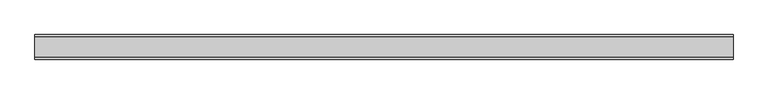
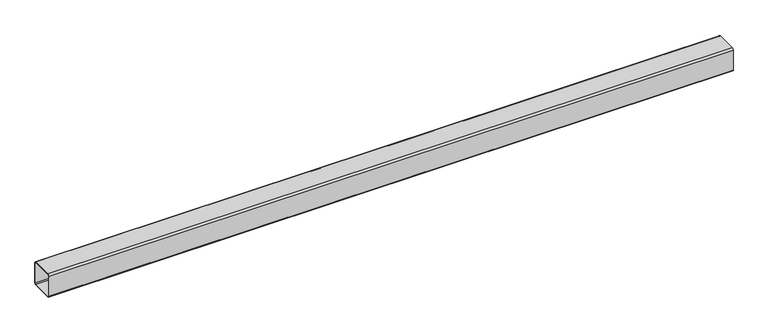
"""IFC4 building model written with IfcOpenShell, lengths in millimetres: beam geometry, Гнутый прямоугольный профиль (Трубы 30245-94) Балки : гнутый прямоуг. проф. 180x6."""

import ifcopenshell
import ifcopenshell.guid

model = None  # the IFC model being written
_history = None  # IfcOwnerHistory: only IFC2X3 demands one
_inside = {}  # id of a spatial element -> (the spatial element, [elements in it])
_under = {}  # id of a project, library or spatial element -> (it, [spatial elements below it])
_declared = {}  # id of a project -> (the project, [libraries it declares])
_typed = {}  # id of a type object -> (the type object, [elements of that type])
_made_of = {}  # id of a material, layer set ... -> (it, [elements and type objects made of it])


def new_model(schema):
    """Start an empty IFC model of exactly this schema.

    Asked for "IFC4X3", IfcOpenShell would pick the latest addendum, in which some entities
    have other attributes; the version numbers below select the first issue.
    IFC2X3 requires an IfcOwnerHistory on every rooted entity: one is made here for all.
    """
    global model, _history
    if schema == "IFC4X3":
        model = ifcopenshell.file(schema_version=(4, 3, 0, 0))
    else:
        model = ifcopenshell.file(schema=schema)
    _inside.clear()
    _under.clear()
    _declared.clear()
    _typed.clear()
    _made_of.clear()
    _history = None
    if model.schema == "IFC2X3":
        org = make("IfcOrganization", Name="unknown")
        user = make(
            "IfcPersonAndOrganization",
            ThePerson=make("IfcPerson", FamilyName="unknown"),
            TheOrganization=org,
        )
        app = make(
            "IfcApplication",
            ApplicationDeveloper=org,
            Version="unknown",
            ApplicationFullName="unknown",
            ApplicationIdentifier="unknown",
        )
        _history = make(
            "IfcOwnerHistory",
            OwningUser=user,
            OwningApplication=app,
            ChangeAction="ADDED",
            CreationDate=0,
        )
    return model


def make(cls, **values):
    """One entity of the class cls with the attributes given. An attribute that is None is left unset."""
    return model.create_entity(
        cls, **{name: value for name, value in values.items() if value is not None}
    )


def rooted(cls, **values):
    """An entity with a GlobalId (a new one), such as an element, a storey or a relation."""
    return make(cls, GlobalId=ifcopenshell.guid.new(), OwnerHistory=_history, **values)


def si_unit(unit_type, name, prefix=None):
    """IfcSIUnit, for example si_unit("LENGTHUNIT", "METRE", prefix="MILLI")."""
    return make("IfcSIUnit", UnitType=unit_type, Prefix=prefix, Name=name)


def assignment(units):
    """IfcUnitAssignment: the units of a project."""
    return None if units is None else make("IfcUnitAssignment", Units=units)


def point(xyz):
    """IfcCartesianPoint."""
    return None if xyz is None else make("IfcCartesianPoint", Coordinates=xyz)


def direction(xyz):
    """IfcDirection."""
    return None if xyz is None else make("IfcDirection", DirectionRatios=xyz)


def frame(location, z_axis=None, x_axis=None):
    """IfcAxis2Placement3D, a coordinate frame: its origin and axes. An axis left out is left unset."""
    return make(
        "IfcAxis2Placement3D",
        Location=point(location),
        Axis=direction(z_axis),
        RefDirection=direction(x_axis),
    )


def frame_2d(location, x_axis=None):
    """IfcAxis2Placement2D, a coordinate frame in the plane: its origin and x axis."""
    return make(
        "IfcAxis2Placement2D", Location=point(location), RefDirection=direction(x_axis)
    )


def origin():
    """The frame at (0, 0, 0) with its axes left unset."""
    return frame((0.0, 0.0, 0.0))


def place(relative_to, where):
    """IfcLocalPlacement: puts the frame where relative to a parent placement (None: the world)."""
    return make(
        "IfcLocalPlacement", PlacementRelTo=relative_to, RelativePlacement=where
    )


def context(
    kind, dimensions, precision=None, world=None, true_north=None, identifier=None
):
    """IfcGeometricRepresentationContext, for example the 3D "Model" context."""
    return make(
        "IfcGeometricRepresentationContext",
        ContextIdentifier=identifier,
        ContextType=kind,
        CoordinateSpaceDimension=dimensions,
        Precision=precision,
        WorldCoordinateSystem=world,
        TrueNorth=true_north,
    )


def project(units=None, contexts=None):
    """IfcProject with its units and contexts."""
    return rooted(
        "IfcProject",
        Name="project",
        RepresentationContexts=contexts,
        UnitsInContext=assignment(units),
    )


def spatial(cls, under=None, at=None, **own):
    """A site, building, storey or space (cls), placed at a placement, below another one or the project."""
    s = rooted(cls, ObjectPlacement=at, **own)
    if under is not None:
        _under.setdefault(under.id(), (under, []))[1].append(s)
    return s


def polyline(points):
    """IfcPolyline through the points."""
    return make("IfcPolyline", Points=[point(p) for p in points])


def circle_curve(where, radius):
    """IfcCircle in the frame where."""
    return make("IfcCircle", Position=where, Radius=radius)


def trimmed(basis, trim1, trim2, sense, master):
    """IfcTrimmedCurve: the piece of a basis curve between two trims."""
    return make(
        "IfcTrimmedCurve",
        BasisCurve=basis,
        Trim1=trim1,
        Trim2=trim2,
        SenseAgreement=sense,
        MasterRepresentation=master,
    )


def segment(curve, same_sense, transition):
    """IfcCompositeCurveSegment."""
    return make(
        "IfcCompositeCurveSegment",
        Transition=transition,
        SameSense=same_sense,
        ParentCurve=curve,
    )


def composite_curve(segments, self_intersect=None):
    """IfcCompositeCurve: segments joined end to end."""
    return make("IfcCompositeCurve", Segments=segments, SelfIntersect=self_intersect)


def outline(outer, holes=None, kind="AREA"):
    """IfcArbitraryClosedProfileDef: a profile drawn as a closed curve; with holes, ...WithVoids."""
    if holes is None:
        return make("IfcArbitraryClosedProfileDef", ProfileType=kind, OuterCurve=outer)
    return make(
        "IfcArbitraryProfileDefWithVoids",
        ProfileType=kind,
        OuterCurve=outer,
        InnerCurves=holes,
    )


def extrude(swept, where, along, depth):
    """IfcExtrudedAreaSolid: the profile swept, set in the frame where, extruded along a direction by depth."""
    return make(
        "IfcExtrudedAreaSolid",
        SweptArea=swept,
        Position=where,
        ExtrudedDirection=direction(along),
        Depth=depth,
    )


def shape(context_of_items, identifier, shape_type, items):
    """IfcShapeRepresentation: the items that make up one representation, for example the "Body"."""
    return make(
        "IfcShapeRepresentation",
        ContextOfItems=context_of_items,
        RepresentationIdentifier=identifier,
        RepresentationType=shape_type,
        Items=items,
    )


def source(mapping_origin, context_of_items, identifier, shape_type, items):
    """IfcRepresentationMap: a shape defined once, which mapped items show again and again."""
    return make(
        "IfcRepresentationMap",
        MappingOrigin=mapping_origin,
        MappedRepresentation=shape(context_of_items, identifier, shape_type, items),
    )


def transform(
    local_origin,
    x_axis=None,
    y_axis=None,
    z_axis=None,
    scale=None,
    scale2=None,
    scale3=None,
    uniform=True,
):
    """IfcCartesianTransformationOperator3D, or its non-uniform kind. x_axis, y_axis, z_axis: its Axis1, 2, 3."""
    if uniform:
        return make(
            "IfcCartesianTransformationOperator3D",
            Axis1=direction(x_axis),
            Axis2=direction(y_axis),
            LocalOrigin=point(local_origin),
            Scale=scale,
            Axis3=direction(z_axis),
        )
    return make(
        "IfcCartesianTransformationOperator3DnonUniform",
        Axis1=direction(x_axis),
        Axis2=direction(y_axis),
        LocalOrigin=point(local_origin),
        Scale=scale,
        Axis3=direction(z_axis),
        Scale2=scale2,
        Scale3=scale3,
    )


def mapped(mapping_source, mapping_target):
    """IfcMappedItem: shows the shape of a source again, moved by a transform."""
    return make(
        "IfcMappedItem", MappingSource=mapping_source, MappingTarget=mapping_target
    )


def made_of(thing, what):
    """Note that an element or type object is made of a material, layer set ...; save() writes the relation."""
    if what is not None:
        _made_of.setdefault(what.id(), (what, []))[1].append(thing)
    return thing


def element(
    cls,
    number,
    at=None,
    inside=None,
    cuts=None,
    type_object=None,
    material=None,
    context=None,
    identifier="Body",
    shape_type=None,
    held_by="IfcProductDefinitionShape",
    body=None,
    shapes=None,
    **own,
):
    """One element of the class cls, such as IfcWall. Its Tag is "e" and its number.

    at: its placement. inside: the storey or other place that contains it. cuts: it is an
    opening in that element (IfcRelVoidsElement). A single representation is given by context,
    identifier, shape_type and body (its items); several are given by shapes. held_by: the class
    of the entity that holds the representations. save() writes the other relations.
    """
    e = rooted(cls, Tag="e%d" % number, ObjectPlacement=at, **own)
    if body is not None:
        shapes = [shape(context, identifier, shape_type, body)]
    if shapes is not None:
        e.Representation = make(held_by, Representations=shapes)
    if inside is not None:
        _inside.setdefault(inside.id(), (inside, []))[1].append(e)
    if cuts is not None:
        rooted(
            "IfcRelVoidsElement", RelatingBuildingElement=cuts, RelatedOpeningElement=e
        )
    if type_object is not None:
        _typed.setdefault(type_object.id(), (type_object, []))[1].append(e)
    return made_of(e, material)


def aggregate(whole, parts):
    """IfcRelAggregates: a whole, such as a stair, and the parts it consists of."""
    return rooted("IfcRelAggregates", RelatingObject=whole, RelatedObjects=parts)


def save(model, path):
    """Write the relations noted so far, then the file.

    IfcRelAggregates (storeys below a building ...), IfcRelContainedInSpatialStructure (elements
    in a storey), IfcRelDefinesByType, IfcRelAssociatesMaterial and IfcRelDeclares: one each for
    every whole, place, type object, material and project.
    """
    for whole, parts in _under.values():
        aggregate(whole, parts)
    for where, things in _inside.values():
        rooted(
            "IfcRelContainedInSpatialStructure",
            RelatedElements=things,
            RelatingStructure=where,
        )
    for kind, things in _typed.values():
        rooted("IfcRelDefinesByType", RelatedObjects=things, RelatingType=kind)
    for what, things in _made_of.values():
        rooted("IfcRelAssociatesMaterial", RelatedObjects=things, RelatingMaterial=what)
    for by, libraries in _declared.values():
        rooted("IfcRelDeclares", RelatingContext=by, RelatedDefinitions=libraries)
    model.write(path)


def beam_75da4e79(model_context):
    return source(origin(), model_context, "Body", "SweptSolid", [
        extrude(outline(composite_curve([segment(polyline([(-78.0, 90.0), (78.0, 90.0)]), True, "CONTINUOUS"), segment(trimmed(circle_curve(frame_2d((78.0, 78.0)), 12.0), [point((78.0, 90.0))], [point((90.0, 78.0))], False, "CARTESIAN"), True, "CONTINUOUS"), segment(polyline([(90.0, 78.0), (90.0, -78.0)]), True, "CONTINUOUS"), segment(trimmed(circle_curve(frame_2d((78.0, -78.0)), 12.0), [point((90.0, -78.0))], [point((78.0, -90.0))], False, "CARTESIAN"), True, "CONTINUOUS"), segment(polyline([(78.0, -90.0), (-78.0, -90.0)]), True, "CONTINUOUS"), segment(trimmed(circle_curve(frame_2d((-78.0, -78.0)), 12.0), [point((-78.0, -90.0))], [point((-90.0, -78.0))], False, "CARTESIAN"), True, "CONTINUOUS"), segment(polyline([(-90.0, -78.0), (-90.0, 78.0)]), True, "CONTINUOUS"), segment(trimmed(circle_curve(frame_2d((-78.0, 78.0)), 12.0), [point((-90.0, 78.0))], [point((-78.0, 90.0))], False, "CARTESIAN"), True, "CONTINUOUS")], self_intersect=False), holes=[composite_curve([segment(trimmed(circle_curve(frame_2d((-78.0, 78.0)), 6.0), [point((-78.0, 84.0))], [point((-84.0, 78.0))], True, "CARTESIAN"), True, "CONTINUOUS"), segment(polyline([(-84.0, 78.0), (-84.0, -78.0)]), True, "CONTINUOUS"), segment(trimmed(circle_curve(frame_2d((-78.0, -78.0)), 6.0), [point((-84.0, -78.0))], [point((-78.0, -84.0))], True, "CARTESIAN"), True, "CONTINUOUS"), segment(polyline([(-78.0, -84.0), (78.0, -84.0)]), True, "CONTINUOUS"), segment(trimmed(circle_curve(frame_2d((78.0, -78.0)), 6.0), [point((78.0, -84.0))], [point((84.0, -78.0))], True, "CARTESIAN"), True, "CONTINUOUS"), segment(polyline([(84.0, -78.0), (84.0, 78.0)]), True, "CONTINUOUS"), segment(trimmed(circle_curve(frame_2d((78.0, 78.0)), 6.0), [point((84.0, 78.0))], [point((78.0, 84.0))], True, "CARTESIAN"), True, "CONTINUOUS"), segment(polyline([(78.0, 84.0), (-78.0, 84.0)]), True, "CONTINUOUS")], self_intersect=False)]), frame((-2550.0, 0.0, 0.0), z_axis=(1.0, 0.0, 0.0), x_axis=(0.0, 1.0, 0.0)), (0.0, 0.0, 1.0), 5100.0),
    ])


if __name__ == "__main__":
    model = new_model("IFC4")
    model_context = context("Model", 3, world=origin())
    ifc_project = project(units=[si_unit("LENGTHUNIT", "METRE", prefix="MILLI")], contexts=[model_context])
    site = spatial("IfcSite", under=ifc_project)
    building = spatial("IfcBuilding", under=site)
    placement = place(None, origin())
    beam_shape = beam_75da4e79(model_context)
    element("IfcBeam", 1, ObjectType="Гнутый прямоугольный профиль (Трубы 30245-94) Балки : гнутый прямоуг. проф. 180x6", at=placement, inside=building, context=model_context, shape_type="MappedRepresentation", body=[
        mapped(beam_shape, transform((0.0, 0.0, 0.0), x_axis=(1.0, 0.0, 0.0), y_axis=(0.0, 1.0, 0.0), z_axis=(0.0, 0.0, 1.0))),
    ])
    save(model, "model.ifc")

# Revit data of these elements
# Type "Гнутый прямоугольный профиль (Трубы 30245-94) Балки : гнутый прямоуг. проф. 180x6"
#   ri = 12 mm
#   ra = 6 mm
#   W = 0.318716
#   Vz = 90 mm
#   Vy = 90 mm
#   Vpz = 90 mm
#   Vpy = 90 mm
#   Length [instance default] = 1500 mm
#   bf = 180 mm
#   d = 180 mm
#   tf = 6 mm
#   tw = 6 mm
#   A = 0.00414 m²
#   Structural Material [instance default] = Металл - Сталь - 345 МПa
#   Assembly Code = ""
# Element 1 (IfcBeam, "Гнутый прямоугольный профиль (Трубы 30245-94) Балки : гнутый прямоуг. проф. 180x6")
#   Structural Material = C245
#   Materials on its faces: "C245"
# Materials
#   "Металл - Сталь - 345 МПa": class "Металл", colour RGB 247 247 247, transparency 0
#   "C245": class "Не назначено", colour RGB 0 0 0, transparency 0
